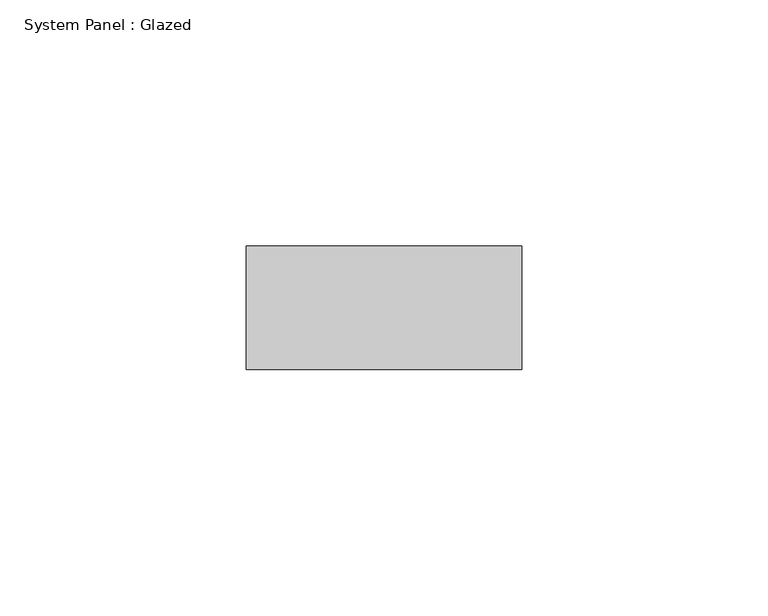
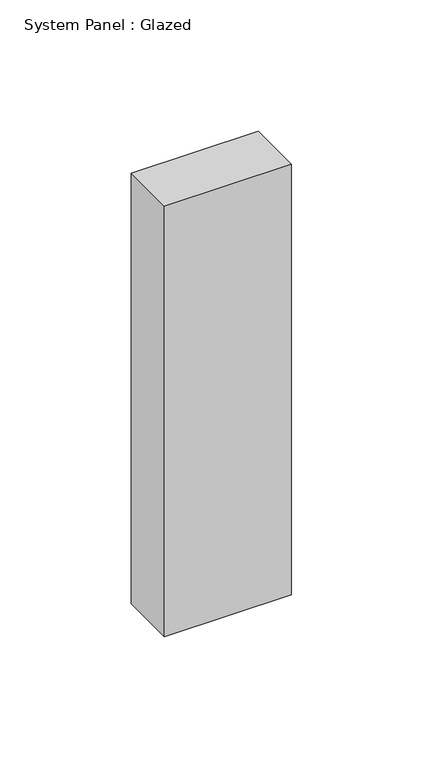
"""IFC4 building model written with IfcOpenShell, lengths in millimetres: plate geometry, System Panel : Glazed."""

from ifc_helpers import new_model, si_unit, origin, origin_with_axes, place, context, project, spatial, polyline, outline, extrude, source, transform, mapped, element, save


def system_panel_glazed_77252c6e(model_context):
    return source(origin(), model_context, "Body", "SweptSolid", [
        extrude(outline(polyline([(27.919021, 24.5), (-27.919021, 24.5), (-27.919021, 49.5), (27.919021, 49.5), (27.919021, 24.5)])), origin_with_axes(), (0.0, 0.0, 1.0), 200.0),
    ])


if __name__ == "__main__":
    model = new_model("IFC4")
    model_context = context("Model", 3, world=origin())
    ifc_project = project(units=[si_unit("LENGTHUNIT", "METRE", prefix="MILLI")], contexts=[model_context])
    site = spatial("IfcSite", under=ifc_project)
    building = spatial("IfcBuilding", under=site)
    placement = place(None, origin())
    system_panel_glazed_shape = system_panel_glazed_77252c6e(model_context)
    element("IfcPlate", 1, ObjectType="System Panel : Glazed", at=placement, inside=building, context=model_context, shape_type="MappedRepresentation", body=[
        mapped(system_panel_glazed_shape, transform((0.0, 0.0, 0.0), x_axis=(1.0, 0.0, 0.0), y_axis=(0.0, 1.0, 0.0), z_axis=(0.0, 0.0, 1.0))),
    ])
    save(model, "model.ifc")

# Revit data of these elements
# Element 1 (IfcPlate, "System Panel : Glazed")
#   Materials on its faces: "Glass"
# Materials
#   "Glass": class "Glass", colour RGB 218 227 224, transparency 0.85, Description = "Soda Lime Glass", Cost = 0
